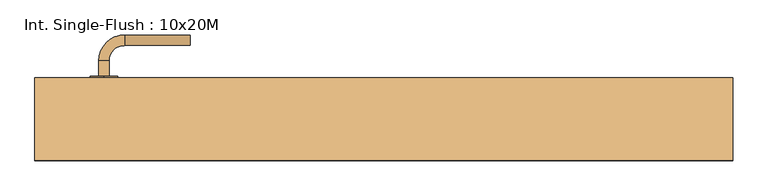
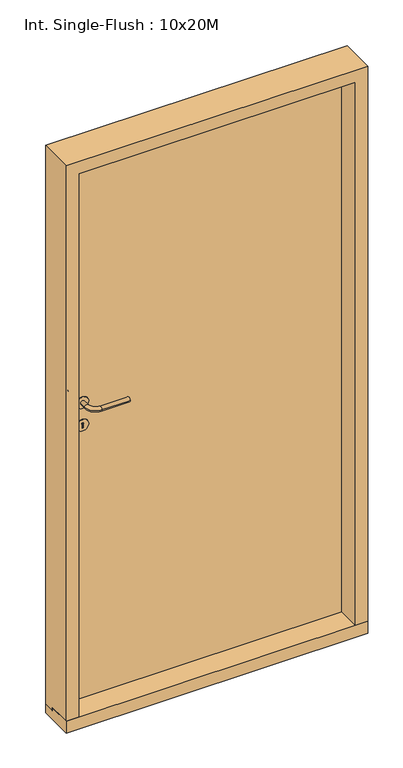
"""IFC4 building model written with IfcOpenShell, lengths in millimetres: door geometry, Int. Single-Flush : 10x20M."""

from ifc_helpers import new_model, si_unit, point, frame, frame_2d, origin, place, context, project, spatial, polyline, circle_curve, ellipse_curve, trimmed, segment, composite_curve, outline, extrude, faceted_brep, source, transform, mapped, element, save
from ifc_brep_helpers import plane_surface, cylinder_surface, revolved_surface, advanced_brep


def int_single_flush_10x20m_e84bf50b(model_context):
    return source(origin(), model_context, "Body", "SolidModel", [
        extrude(outline(composite_curve([segment(trimmed(circle_curve(frame_2d((1090.0, -406.0)), 20.0), [point((1070.0, -406.0))], [point((1110.0, -406.0))], False, "CARTESIAN"), True, "CONTINUOUS"), segment(trimmed(circle_curve(frame_2d((1090.0, -406.0)), 20.0), [point((1110.0, -406.0))], [point((1070.0, -406.0))], False, "CARTESIAN"), True, "CONTINUOUS")], self_intersect=False)), frame((0.0, 60.0, 0.0), z_axis=(0.0, 1.0, 0.0), x_axis=(0.0, 0.0, 1.0)), (0.0, 0.0, 1.0), 2.0),
        advanced_brep(
        [(-413.5, 62.0, 1090.0), (-398.5, 62.0, 1090.0), (-413.5, 84.5, 1090.0), (-398.5, 84.5, 1090.0), (-376.0, 107.0, 1090.0), (-376.0, 122.0, 1090.0), (-281.0, 122.0, 1090.0), (-281.0, 107.0, 1090.0)],
        [
            (0, 1, circle_curve(frame((-406.0, 62.0, 1090.0), z_axis=(0.0, -1.0, 0.0), x_axis=(1.0, 0.0, 0.0)), 7.5)),
            (1, 0, circle_curve(frame((-406.0, 62.0, 1090.0), z_axis=(0.0, -1.0, 0.0), x_axis=(1.0, 0.0, 0.0)), 7.5)),
            (0, 2),
            (2, 3, circle_curve(frame((-406.0, 84.5, 1090.0), z_axis=(0.0, -1.0, 0.0), x_axis=(1.0, 0.0, 0.0)), 7.5)),
            (3, 1),
            (3, 2, circle_curve(frame((-406.0, 84.5, 1090.0), z_axis=(0.0, -1.0, 0.0), x_axis=(1.0, 0.0, 0.0)), 7.5)),
            (4, 3, circle_curve(frame((-376.0, 84.5, 1090.0), z_axis=(0.0, 0.0, 1.0), x_axis=(-1.0, 0.0, 0.0)), 22.5)),
            (2, 5, circle_curve(frame((-376.0, 84.5, 1090.0), z_axis=(0.0, 0.0, -1.0), x_axis=(-1.0, 0.0, 0.0)), 37.5)),
            (5, 4, circle_curve(frame((-376.0, 114.5, 1090.0), z_axis=(-1.0, 0.0, 0.0), x_axis=(0.0, -1.0, 0.0)), 7.5)),
            (4, 5, circle_curve(frame((-376.0, 114.5, 1090.0), z_axis=(-1.0, 0.0, 0.0), x_axis=(0.0, -1.0, 0.0)), 7.5)),
            (5, 6),
            (6, 7, circle_curve(frame((-281.0, 114.5, 1090.0), z_axis=(-1.0, 0.0, 0.0), x_axis=(0.0, -1.0, 0.0)), 7.5)),
            (7, 4),
            (7, 6, circle_curve(frame((-281.0, 114.5, 1090.0), z_axis=(-1.0, 0.0, 0.0), x_axis=(0.0, -1.0, 0.0)), 7.5)),
        ],
        [
            plane_surface(frame((-406.0, 62.0, 1090.0), z_axis=(0.0, -1.0, 0.0), x_axis=(0.0, 0.0, -1.0))),
            cylinder_surface(frame((-406.0, 62.0, 1090.0), z_axis=(0.0, -1.0, 0.0), x_axis=(1.0, 0.0, 0.0)), 7.5),
            revolved_surface(trimmed(ellipse_curve(frame((-406.0, 84.5, 1090.0), z_axis=(0.0, -1.0, 0.0), x_axis=(1.0, 0.0, 0.0)), 7.5, 7.5), [point((-413.5, 84.5, 1090.0))], [point((-398.5, 84.5, 1090.0))], True, "CARTESIAN"), (-376.0, 84.5, 1090.0), (0.0, 0.0, -1.0)),
            revolved_surface(trimmed(ellipse_curve(frame((-406.0, 84.5, 1090.0), z_axis=(0.0, -1.0, 0.0), x_axis=(1.0, 0.0, 0.0)), 7.5, 7.5), [point((-398.5, 84.5, 1090.0))], [point((-413.5, 84.5, 1090.0))], True, "CARTESIAN"), (-376.0, 84.5, 1090.0), (0.0, 0.0, -1.0)),
            cylinder_surface(frame((-376.0, 114.5, 1090.0), z_axis=(-1.0, 0.0, 0.0), x_axis=(0.0, -1.0, 0.0)), 7.5),
            plane_surface(frame((-281.0, 114.5, 1090.0), z_axis=(1.0, 0.0, 0.0), x_axis=(0.0, 0.0, -1.0))),
        ],
        [
            (0, [[1, 2]]),
            (1, [[-1, 3, 4, 5]]),
            (1, [[-2, -5, 6, -3]]),
            (2, [[7, -4, 8, 9]]),
            (3, [[-8, -6, -7, 10]]),
            (4, [[-9, 11, 12, 13]]),
            (4, [[-10, -13, 14, -11]]),
            (5, [[-14, -12]]),
        ],
    ),
        extrude(outline(composite_curve([segment(trimmed(circle_curve(frame_2d((1010.0, -406.0)), 20.0), [point((990.0, -406.0))], [point((1030.0, -406.0))], False, "CARTESIAN"), True, "CONTINUOUS"), segment(trimmed(circle_curve(frame_2d((1010.0, -406.0)), 20.0), [point((1030.0, -406.0))], [point((990.0, -406.0))], False, "CARTESIAN"), True, "CONTINUOUS")], self_intersect=False), holes=[composite_curve([segment(trimmed(circle_curve(frame_2d((1015.0, -406.0)), 3.0), [point((1012.4019238, -407.5))], [point((1012.4019238, -404.5))], True, "CARTESIAN"), True, "CONTINUOUS"), segment(polyline([(1012.4019238, -404.5), (1000.0, -404.5), (1000.0, -407.5), (1012.4019238, -407.5)]), True, "CONTINUOUS")], self_intersect=False)]), frame((0.0, 60.0, 0.0), z_axis=(0.0, 1.0, 0.0), x_axis=(0.0, 0.0, 1.0)), (0.0, 0.0, 1.0), 2.0),
        extrude(outline(composite_curve([segment(trimmed(circle_curve(frame_2d((1090.0, -406.0)), 20.0), [point((1070.0, -406.0))], [point((1110.0, -406.0))], False, "CARTESIAN"), True, "CONTINUOUS"), segment(trimmed(circle_curve(frame_2d((1090.0, -406.0)), 20.0), [point((1110.0, -406.0))], [point((1070.0, -406.0))], False, "CARTESIAN"), True, "CONTINUOUS")], self_intersect=False)), frame((0.0, 18.0, 0.0), z_axis=(0.0, 1.0, 0.0), x_axis=(0.0, 0.0, 1.0)), (0.0, 0.0, 1.0), 2.0),
        advanced_brep(
        [(-413.5, 18.0, 1090.0), (-398.5, 18.0, 1090.0), (-398.5, -4.5, 1090.0), (-413.5, -4.5, 1090.0), (-376.0, -27.0, 1090.0), (-376.0, -42.0, 1090.0), (-281.0, -27.0, 1090.0), (-281.0, -42.0, 1090.0)],
        [
            (0, 1, circle_curve(frame((-406.0, 18.0, 1090.0), z_axis=(0.0, 1.0, 0.0), x_axis=(1.0, 0.0, 0.0)), 7.5)),
            (1, 0, circle_curve(frame((-406.0, 18.0, 1090.0), z_axis=(0.0, 1.0, 0.0), x_axis=(1.0, 0.0, 0.0)), 7.5)),
            (1, 2),
            (2, 3, circle_curve(frame((-406.0, -4.5, 1090.0), z_axis=(0.0, 1.0, 0.0), x_axis=(1.0, 0.0, 0.0)), 7.5)),
            (3, 0),
            (3, 2, circle_curve(frame((-406.0, -4.5, 1090.0), z_axis=(0.0, 1.0, 0.0), x_axis=(1.0, 0.0, 0.0)), 7.5)),
            (4, 5, circle_curve(frame((-376.0, -34.5, 1090.0), z_axis=(-1.0, 0.0, 0.0), x_axis=(0.0, 1.0, 0.0)), 7.5)),
            (5, 3, circle_curve(frame((-376.0, -4.5, 1090.0), z_axis=(0.0, 0.0, -1.0), x_axis=(-1.0, 0.0, 0.0)), 37.5)),
            (2, 4, circle_curve(frame((-376.0, -4.5, 1090.0), z_axis=(0.0, 0.0, 1.0), x_axis=(-1.0, 0.0, 0.0)), 22.5)),
            (5, 4, circle_curve(frame((-376.0, -34.5, 1090.0), z_axis=(-1.0, 0.0, 0.0), x_axis=(0.0, 1.0, 0.0)), 7.5)),
            (4, 6),
            (6, 7, circle_curve(frame((-281.0, -34.5, 1090.0), z_axis=(-1.0, 0.0, 0.0), x_axis=(0.0, 1.0, 0.0)), 7.5)),
            (7, 5),
            (7, 6, circle_curve(frame((-281.0, -34.5, 1090.0), z_axis=(-1.0, 0.0, 0.0), x_axis=(0.0, 1.0, 0.0)), 7.5)),
        ],
        [
            plane_surface(frame((-406.0, 18.0, 1090.0), z_axis=(0.0, 1.0, 0.0), x_axis=(0.0, 0.0, -1.0))),
            cylinder_surface(frame((-406.0, 18.0, 1090.0), z_axis=(0.0, 1.0, 0.0), x_axis=(1.0, 0.0, 0.0)), 7.5),
            revolved_surface(trimmed(ellipse_curve(frame((-406.0, -4.5, 1090.0), z_axis=(0.0, -1.0, 0.0), x_axis=(1.0, 0.0, 0.0)), 7.5, 7.5), [point((-413.5, -4.5, 1090.0))], [point((-398.5, -4.5, 1090.0))], True, "CARTESIAN"), (-376.0, -4.5, 1090.0), (0.0, 0.0, -1.0)),
            revolved_surface(trimmed(ellipse_curve(frame((-406.0, -4.5, 1090.0), z_axis=(0.0, -1.0, 0.0), x_axis=(1.0, 0.0, 0.0)), 7.5, 7.5), [point((-398.5, -4.5, 1090.0))], [point((-413.5, -4.5, 1090.0))], True, "CARTESIAN"), (-376.0, -4.5, 1090.0), (0.0, 0.0, -1.0)),
            cylinder_surface(frame((-376.0, -34.5, 1090.0), z_axis=(-1.0, 0.0, 0.0), x_axis=(0.0, 1.0, 0.0)), 7.5),
            plane_surface(frame((-281.0, -34.5, 1090.0), z_axis=(1.0, 0.0, 0.0), x_axis=(0.0, 0.0, -1.0))),
        ],
        [
            (0, [[1, 2]]),
            (1, [[3, 4, 5, -2]]),
            (1, [[-5, 6, -3, -1]]),
            (2, [[7, 8, -4, 9]]),
            (3, [[10, -9, -6, -8]]),
            (4, [[11, 12, 13, -7]]),
            (4, [[-13, 14, -11, -10]]),
            (5, [[-12, -14]]),
        ],
    ),
        extrude(outline(composite_curve([segment(trimmed(circle_curve(frame_2d((1010.0, -406.0)), 20.0), [point((990.0, -406.0))], [point((1030.0, -406.0))], False, "CARTESIAN"), True, "CONTINUOUS"), segment(trimmed(circle_curve(frame_2d((1010.0, -406.0)), 20.0), [point((1030.0, -406.0))], [point((990.0, -406.0))], False, "CARTESIAN"), True, "CONTINUOUS")], self_intersect=False), holes=[composite_curve([segment(trimmed(circle_curve(frame_2d((1015.0, -406.0)), 3.0), [point((1012.4019238, -407.5))], [point((1012.4019238, -404.5))], True, "CARTESIAN"), True, "CONTINUOUS"), segment(polyline([(1012.4019238, -404.5), (1000.0, -404.5), (1000.0, -407.5), (1012.4019238, -407.5)]), True, "CONTINUOUS")], self_intersect=False)]), frame((0.0, 18.0, 0.0), z_axis=(0.0, 1.0, 0.0), x_axis=(0.0, 0.0, 1.0)), (0.0, 0.0, 1.0), 2.0),
        extrude(outline(polyline([(476.0, 20.0), (-476.0, 20.0), (-476.0, 60.0), (476.0, 60.0), (476.0, 20.0)])), frame((0.0, 0.0, 30.0), z_axis=(0.0, 0.0, 1.0), x_axis=(1.0, 0.0, 0.0)), (0.0, 0.0, 1.0), 1952.0),
        extrude(outline(polyline([(20.0, 42.0), (20.0, 30.0), (60.0, 30.0), (60.0, 0.0), (-60.0, 0.0), (-60.0, 42.0), (20.0, 42.0)])), frame((-506.0, 0.0, 0.0), z_axis=(1.0, 0.0, 0.0), x_axis=(0.0, 1.0, 0.0)), (0.0, 0.0, 1.0), 1012.0),
        faceted_brep([(-476.0, 20.0, 1982.0), (476.0, 20.0, 1982.0), (476.0, 20.0, 42.0), (464.0, 20.0, 42.0), (464.0, 20.0, 1970.0), (-464.0, 20.0, 1970.0), (-464.0, 20.0, 42.0), (-476.0, 20.0, 42.0), (-476.0, 60.0, 1982.0), (-476.0, 20.0, 30.0), (-476.0, 60.0, 30.0), (-506.0, 20.0, 42.0), (-506.0, 20.0, 30.0), (506.0, 20.0, 42.0), (476.0, 20.0, 30.0), (506.0, 20.0, 30.0), (-506.0, 60.0, 30.0), (476.0, 60.0, 30.0), (506.0, 60.0, 30.0), (-506.0, 60.0, 2012.0), (506.0, 60.0, 2012.0), (476.0, 60.0, 1982.0), (-464.0, -60.0, 42.0), (-506.0, -60.0, 42.0), (506.0, -60.0, 42.0), (464.0, -60.0, 42.0), (464.0, -60.0, 1970.0), (-464.0, -60.0, 1970.0), (506.0, -60.0, 2012.0), (-506.0, -60.0, 2012.0)], [[[0, 1, 2, 3, 4, 5, 6, 7]], [[8, 0, 7, 9, 10]], [[7, 11, 12, 9]], [[13, 2, 14, 15]], [[9, 12, 16, 10]], [[15, 14, 17, 18]], [[19, 20, 18, 17, 21, 8, 10, 16]], [[1, 21, 17, 14, 2]], [[11, 7, 6, 22, 23]], [[2, 13, 24, 25, 3]], [[26, 4, 3, 25]], [[5, 27, 22, 6]], [[27, 26, 25, 24, 28, 29, 23, 22]], [[20, 28, 24, 13, 15, 18]], [[29, 19, 16, 12, 11, 23]], [[0, 8, 21, 1]], [[5, 4, 26, 27]], [[29, 28, 20, 19]]]),
    ])


if __name__ == "__main__":
    model = new_model("IFC4")
    model_context = context("Model", 3, world=origin())
    ifc_project = project(units=[si_unit("LENGTHUNIT", "METRE", prefix="MILLI")], contexts=[model_context])
    site = spatial("IfcSite", under=ifc_project)
    building = spatial("IfcBuilding", under=site)
    placement = place(None, origin())
    int_single_flush_10x20m_shape = int_single_flush_10x20m_e84bf50b(model_context)
    element("IfcDoor", 1, ObjectType="Int. Single-Flush : 10x20M", at=placement, inside=building, context=model_context, shape_type="MappedRepresentation", body=[
        mapped(int_single_flush_10x20m_shape, transform((0.0, 0.0, 0.0), x_axis=(1.0, 0.0, 0.0), y_axis=(0.0, 1.0, 0.0), z_axis=(0.0, 0.0, 1.0))),
    ])
    save(model, "model.ifc")

# Revit data of these elements
# Type "Int. Single-Flush : 10x20M"
#   Type Mark = "73"
#   Sound Rating = ""
#   Hinge Side [instance default] = ""
#   Creator Organization [instance default] = "© Danish Educational Content"
#   Creator Name [instance default] = "© Erik Falck Jørgensen"
#   Creator Build [instance default] = "2017.0801.0"
#   Analytic Construction = "<None>"
#   length#5 = 1012 mm
#   length#3 = 42 mm
#   length#2b = 12 mm
#   length#2a = 0 mm
#   length#2 = 0 mm
#   length#1a = 12 mm
#   length#1 = 0 mm
#   length#4 = 30 mm
#   Thickness = 40 mm
#   Seal Width = 12 mm
#   Rough Width = 1012 mm
#   Rough Height = 2012 mm
#   Rabbet Depth = 40 mm
#   Interior Distance [instance default] = 0 mm
#   Height = 1988 mm
#   Width = 988 mm
#   Handle From Side = 100 mm
#   Handle From Bottom = 1090 mm
#   Exterior Direction [instance default] = 0.00°
#   Case Depth [instance default] = 200 mm
#   Case Width = 30 mm
#   Rabbet Width = 12 mm
#   Exterior Distance [instance default] = 0 mm
#   Bottom Seal = 12 mm
#   Threshold = yes
#   Sealing = no
#   Hinging = yes
#   Wall Closure = 1
#   Door Panel = no
#   Panel = none
#   Handle Finish = none
#   Handle = element 510752
#   Case/Transom = none
#   Function = (empty or 0)
#   Assembly Code = ""
# Element 1 (IfcDoor, "Int. Single-Flush : 10x20M")
#   Case Depth = 120 mm
#   Materials on its faces: "Stainless Steel, Polished", "Default Frame/Mullion (Interior/Exterior)", "Default Door Panel (Exterior/Interior)"
# Materials
#   "Stainless Steel, Polished": class "Metal", colour RGB 180 180 180, transparency 0, Description = "Rustfri stål, poleret", Cost = 0
#   "Default Frame/Mullion (Interior/Exterior)": class "Generic", colour RGB 205 205 205, transparency 0, Description = "Udefineret karm/ramme materiale", Cost = 0
#   "Default Door Panel (Exterior/Interior)": class "Generic", colour RGB 205 205 205, transparency 0, Description = "Udefineret dørplade materiale", Cost = 0
